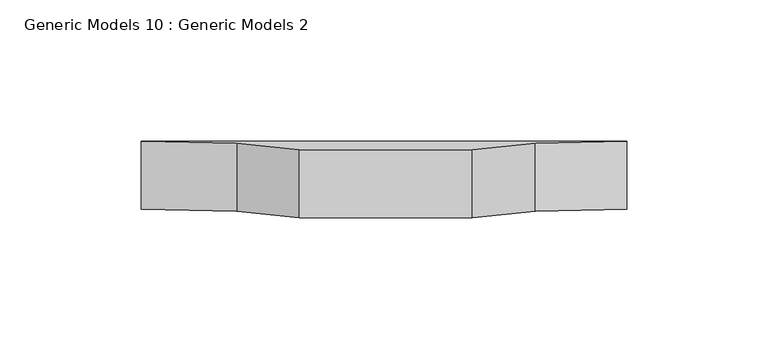
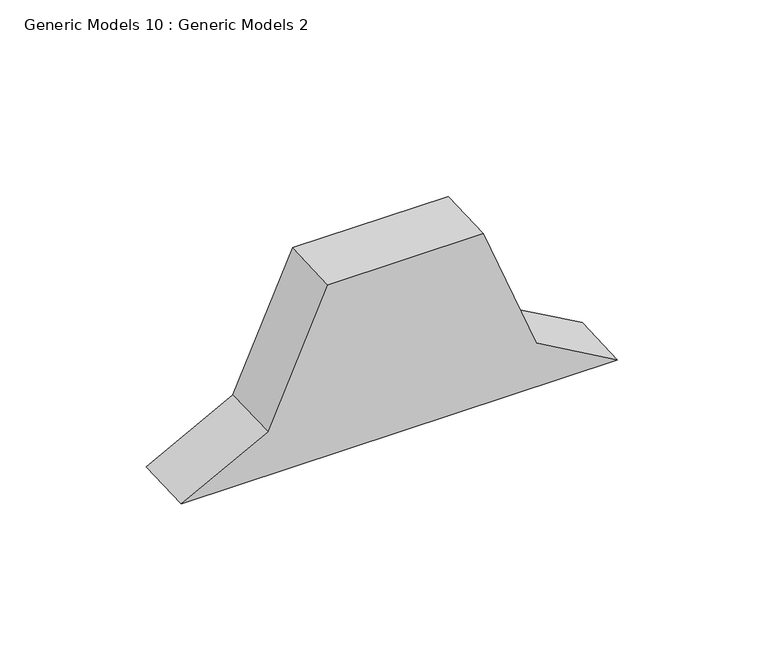
"""IFC4 building model written with IfcOpenShell, lengths in millimetres: proxy geometry, Generic Models 10 : Generic Models 2."""

from ifc_helpers import new_model, si_unit, frame, origin, place, context, project, spatial, polyline, outline, extrude, source, transform, mapped, element, save


def generic_models_10_generic_models_2_fc529abc(model_context):
    return source(origin(), model_context, "Body", "SweptSolid", [
        extrude(outline(polyline([(-38.6882115, -1e-07), (0.0, 0.0), (-150.7153107, -83.4176452), (-131.3348102, -51.2109659), (-138.5264806, 7.6691636), (-84.8134897, 37.3981354), (-38.6882115, -1e-07)])), frame((592834.8996639, -568249.5160673, 8801.076176), z_axis=(0.0, 0.9991330730923521, 0.041630544712176844), x_axis=(-0.8749277528680572, 0.020159735909129006, -0.48383366181914833)), (0.0, 0.0, 1.0), 24.1018037),
    ])


if __name__ == "__main__":
    model = new_model("IFC4")
    model_context = context("Model", 3, world=origin())
    ifc_project = project(units=[si_unit("LENGTHUNIT", "METRE", prefix="MILLI")], contexts=[model_context])
    site = spatial("IfcSite", under=ifc_project)
    building = spatial("IfcBuilding", under=site)
    placement = place(None, origin())
    generic_models_10_generic_models_2_shape = generic_models_10_generic_models_2_fc529abc(model_context)
    element("IfcBuildingElementProxy", 1, Name="Generic Models 10 : Generic Models 2", ObjectType="Generic Models 10 : Generic Models 2", at=placement, inside=building, context=model_context, shape_type="MappedRepresentation", body=[
        mapped(generic_models_10_generic_models_2_shape, transform((0.0, 0.0, 0.0), x_axis=(1.0, 0.0, 0.0), y_axis=(0.0, 1.0, 0.0), z_axis=(0.0, 0.0, 1.0))),
    ])
    save(model, "model.ifc")

# Revit data of these elements
# Element 1 (IfcBuildingElementProxy, "Generic Models 10 : Generic Models 2")
#   Materials on its faces: "METAL CLOSURE AT RIBS AND JOINTS - TAPE SEALER ALONG PERIMETER"
# Materials
#   "METAL CLOSURE AT RIBS AND JOINTS - TAPE SEALER ALONG PERIMETER": class "Generic", colour RGB 117 119 119, transparency 0, Cost = 0
